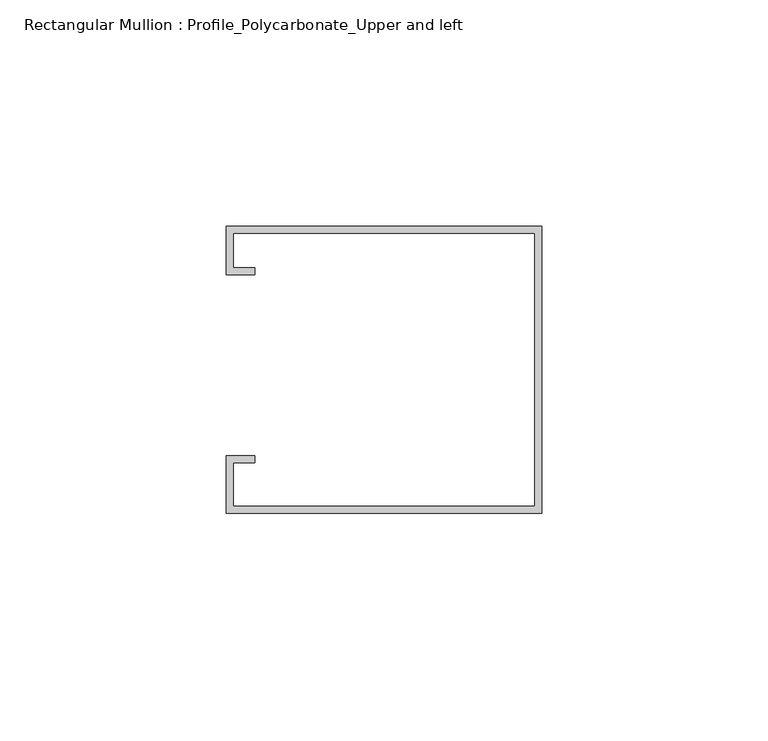
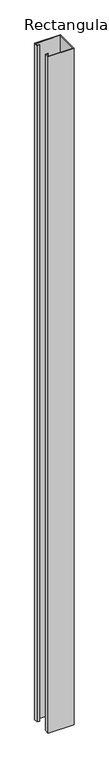
"""IFC4 building model written with IfcOpenShell, lengths in millimetres: member geometry, Rectangular Mullion : Profile_Polycarbonate_Upper and left."""

from ifc_helpers import new_model, si_unit, frame, origin, place, context, project, spatial, polyline, outline, extrude, source, transform, mapped, element, save


def rectangular_mullion_profile_polycarbonate_upper_and_left_327f1905(model_context):
    return source(origin(), model_context, "Body", "SweptSolid", [
        extrude(outline(polyline([(0.0, -32.7), (-69.85, -32.7), (-69.85, -20.0), (-63.5, -20.0), (-63.5, -21.5875), (-68.2625, -21.5875), (-68.2625, -31.1125), (-1.5875, -31.1125), (-1.5875, 29.2125), (-68.2625, 29.2125), (-68.2625, 21.5875), (-63.5, 21.5875), (-63.5, 20.0), (-69.85, 20.0), (-69.85, 30.8), (0.0, 30.8), (0.0, -32.7)])), frame((0.0, 0.0, -1943.1), z_axis=(0.0, 0.0, 1.0), x_axis=(1.0, 0.0, 0.0)), (0.0, 0.0, 1.0), 1943.1),
    ])


if __name__ == "__main__":
    model = new_model("IFC4")
    model_context = context("Model", 3, world=origin())
    ifc_project = project(units=[si_unit("LENGTHUNIT", "METRE", prefix="MILLI")], contexts=[model_context])
    site = spatial("IfcSite", under=ifc_project)
    building = spatial("IfcBuilding", under=site)
    placement = place(None, origin())
    rectangular_mullion_profile_polycarbonate_upper_and_left_shape = rectangular_mullion_profile_polycarbonate_upper_and_left_327f1905(model_context)
    element("IfcMember", 1, ObjectType="Rectangular Mullion : Profile_Polycarbonate_Upper and left", at=placement, inside=building, context=model_context, shape_type="MappedRepresentation", body=[
        mapped(rectangular_mullion_profile_polycarbonate_upper_and_left_shape, transform((0.0, 0.0, 0.0), x_axis=(1.0, 0.0, 0.0), y_axis=(0.0, 1.0, 0.0), z_axis=(0.0, 0.0, 1.0))),
    ])
    save(model, "model.ifc")

# Revit data of these elements
# Type "Rectangular Mullion : Profile_Polycarbonate_Upper and left"
#   built-in parameter 1007322 = 0.208333 (stored number, unit not read)
#   built-in parameter 1007321 = 0.00520833 (stored number, unit not read)
#   built-in parameter 1007320 = 0 (stored number, unit not read)
# Element 1 (IfcMember, "Rectangular Mullion : Profile_Polycarbonate_Upper and left")
#   Materials on its faces: "GALVANIZED UNISTRUT P5500, 1 5/8\" X 2 7/16\" OR ALUM. CHANNEL"
# Materials
#   "GALVANIZED UNISTRUT P5500, 1 5/8\" X 2 7/16\" OR ALUM. CHANNEL": class "Metal", colour RGB 244 244 244, transparency 0, Description = "Aluminum 6061", Cost = 0
